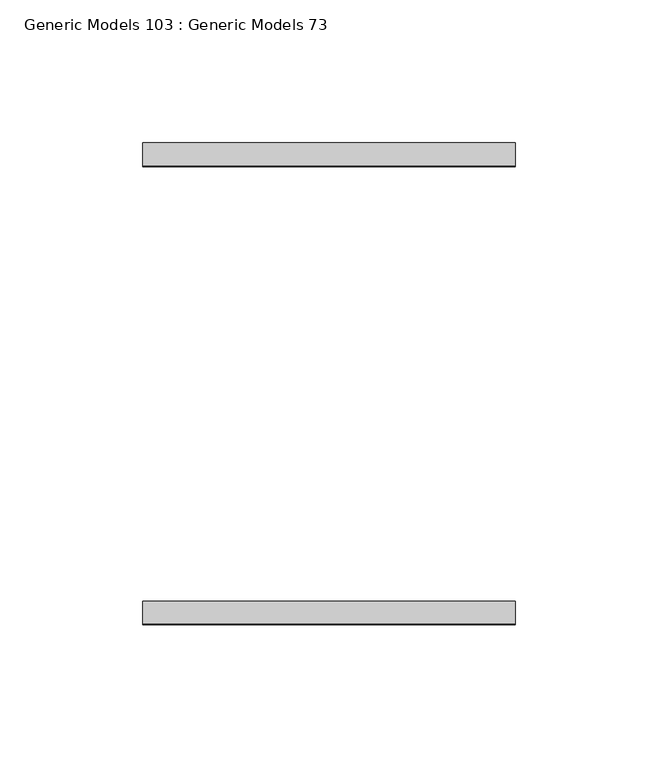
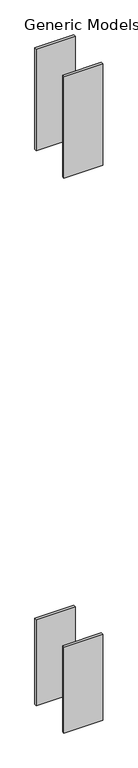
"""IFC4 building model written with IfcOpenShell, lengths in millimetres: proxy geometry, Generic Models 103 : Generic Models 73."""

from ifc_helpers import new_model, si_unit, frame, origin, place, context, project, spatial, polyline, outline, extrude, source, transform, mapped, element, save


def generic_models_103_generic_models_73_86a274db(model_context):
    return source(origin(), model_context, "Body", "SweptSolid", [
        extrude(outline(polyline([(32040.4971032, 30858.4781612), (32040.4971032, 30850.5406612), (31910.3221032, 30850.5406612), (31910.3221032, 30858.4781612), (32040.4971032, 30858.4781612)])), frame((0.0, 0.0, 268388.9485545), z_axis=(0.0, 0.0, 1.0), x_axis=(1.0, 0.0, 0.0)), (0.0, 0.0, 1.0), 360.5139455),
        extrude(outline(polyline([(32040.4971032, 30698.1406612), (32040.4971032, 30690.2031612), (31910.3221032, 30690.2031612), (31910.3221032, 30698.1406612), (32040.4971032, 30698.1406612)])), frame((0.0, 0.0, 268388.9485545), z_axis=(0.0, 0.0, 1.0), x_axis=(1.0, 0.0, 0.0)), (0.0, 0.0, 1.0), 360.5139455),
        extrude(outline(polyline([(32040.4971032, 30858.4781612), (32040.4971032, 30850.5406612), (31910.3221032, 30850.5406612), (31910.3221032, 30858.4781612), (32040.4971032, 30858.4781612)])), frame((0.0, 0.0, 266422.1875), z_axis=(0.0, 0.0, 1.0), x_axis=(1.0, 0.0, 0.0)), (0.0, 0.0, 1.0), 304.8),
        extrude(outline(polyline([(32040.4971032, 30698.1406612), (32040.4971032, 30690.2031612), (31910.3221032, 30690.2031612), (31910.3221032, 30698.1406612), (32040.4971032, 30698.1406612)])), frame((0.0, 0.0, 266422.1875), z_axis=(0.0, 0.0, 1.0), x_axis=(1.0, 0.0, 0.0)), (0.0, 0.0, 1.0), 304.8),
    ])


if __name__ == "__main__":
    model = new_model("IFC4")
    model_context = context("Model", 3, world=origin())
    ifc_project = project(units=[si_unit("LENGTHUNIT", "METRE", prefix="MILLI")], contexts=[model_context])
    site = spatial("IfcSite", under=ifc_project)
    building = spatial("IfcBuilding", under=site)
    placement = place(None, origin())
    generic_models_103_generic_models_73_shape = generic_models_103_generic_models_73_86a274db(model_context)
    element("IfcBuildingElementProxy", 1, Name="Generic Models 103 : Generic Models 73", ObjectType="Generic Models 103 : Generic Models 73", at=placement, inside=building, context=model_context, shape_type="MappedRepresentation", body=[
        mapped(generic_models_103_generic_models_73_shape, transform((0.0, 0.0, 0.0), x_axis=(1.0, 0.0, 0.0), y_axis=(0.0, 1.0, 0.0), z_axis=(0.0, 0.0, 1.0))),
    ])
    save(model, "model.ifc")

# Revit data of these elements
# Element 1 (IfcBuildingElementProxy, "Generic Models 103 : Generic Models 73")
#   Materials on its faces: "5/16 x 5 1/2\" x 1'-0\" SIDE PLATES  CAP\nW/ 2 3/4\"DIA. THRU BOLTS"
# Materials
#   "5/16 x 5 1/2\" x 1'-0\" SIDE PLATES  CAP\nW/ 2 3/4\"DIA. THRU BOLTS": class "Metal", colour RGB 199 199 199, transparency 0, Description = "Carbon steel", Cost = 0
